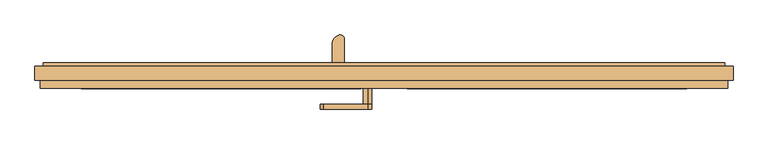
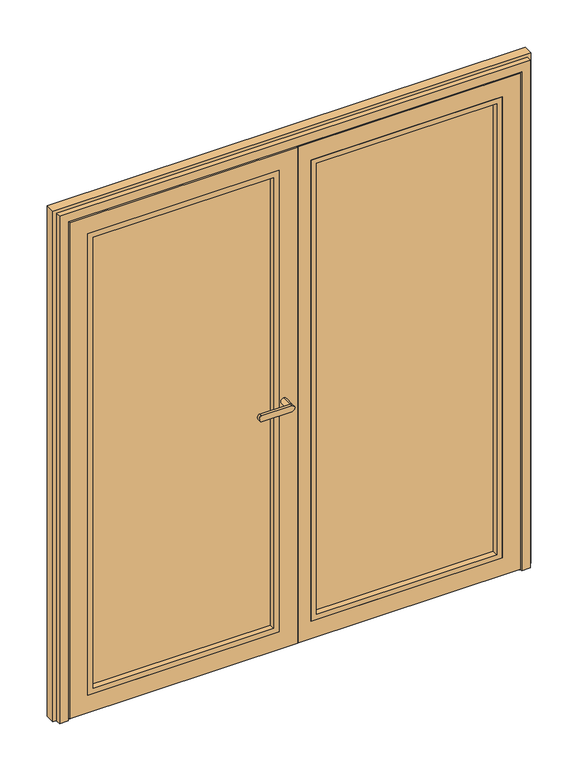
"""IFC4 building model written with IfcOpenShell, lengths in millimetres: door geometry, Schueco_FWS_ADS-70-HD_inw_Family-02 : FWS SI insert unit."""

from ifc_helpers import new_model, si_unit, point, frame, frame_2d, origin, place, context, project, spatial, polyline, circle_curve, ellipse_curve, trimmed, segment, composite_curve, outline, extrude, faceted_brep, source, transform, mapped, element, save
from ifc_brep_helpers import plane_surface, cylinder_surface, extruded_surface, advanced_brep


def door_4fc60986(model_context):
    return source(origin(), model_context, "Body", "SolidModel", [
        faceted_brep([(900.0, -52.5000065, 8.0), (900.0, -52.5000065, 2100.0), (900.0, -61.0002823, 2100.0), (900.0, -61.0002823, 8.0), (15.0, -61.0002823, 8.0), (15.0, -52.5000065, 8.0), (15.0, -52.5000065, 23.0), (885.0, -52.5000065, 23.0), (885.0, -52.5000065, 2085.0), (15.0, -52.5000065, 2085.0), (15.0, -52.5000065, 2100.0), (15.0, -61.0002823, 2100.0), (63.0, -61.0002823, 81.0), (63.0, -61.0002823, 2027.0), (827.0, -61.0002823, 2027.0), (827.0, -61.0002823, 81.0), (827.0, 0.4997603, 2027.0), (827.0, 0.4997603, 81.0), (63.0, 0.4997603, 81.0), (63.0, 0.4997603, 2027.0), (88.0, 0.4997603, 106.0), (88.0, 0.4997603, 2002.0), (802.0, 0.4997603, 2002.0), (802.0, 0.4997603, 106.0), (802.0, 8.9997177, 2002.0), (802.0, 8.9997177, 106.0), (88.0, 8.9997177, 106.0), (88.0, 8.9997177, 2002.0), (875.0, 8.9997177, 33.0), (-10.0, 8.9997177, 33.0), (-10.0, 8.9997177, 2075.0), (875.0, 8.9997177, 2075.0), (875.0, 0.4997603, 2075.0), (875.0, 0.4997603, 33.0), (5.0, 0.4997603, 33.0), (-10.0, 0.4997603, 33.0), (5.0, 0.4997603, 23.0), (5.0, 0.4997603, 2075.0), (5.0, 0.4997603, 2085.0), (885.0, 0.4997603, 2085.0), (885.0, 0.4997603, 23.0), (5.0, -52.5000065, 23.0), (5.0, -52.5000065, 2085.0), (-10.0, 0.4997603, 2075.0)], [[[0, 1, 2, 3]], [[3, 4, 5, 0]], [[0, 5, 6, 7, 8, 9, 10, 1]], [[2, 11, 4, 3], [12, 13, 14, 15]], [[15, 14, 16, 17]], [[17, 18, 12, 15]], [[18, 19, 13, 12]], [[17, 16, 19, 18], [20, 21, 22, 23]], [[23, 22, 24, 25]], [[25, 26, 20, 23]], [[26, 27, 21, 20]], [[28, 29, 30, 31], [25, 24, 27, 26]], [[28, 31, 32, 33]], [[33, 34, 35, 29, 28]], [[36, 34, 33, 32, 37, 38, 39, 40]], [[40, 39, 8, 7]], [[7, 6, 41, 36, 40]], [[41, 42, 38, 37, 34, 36]], [[1, 10, 11, 2]], [[19, 16, 14, 13]], [[27, 24, 22, 21]], [[31, 30, 43, 37, 32]], [[42, 9, 8, 39, 38]], [[6, 5, 4, 11, 10, 9]], [[35, 43, 30, 29]], [[35, 34, 37, 43]], [[9, 42, 41, 6]]]),
        extrude(outline(polyline([(81.0, 63.0), (81.0, 827.0), (2027.0, 827.0), (2027.0, 63.0), (81.0, 63.0)]), holes=[polyline([(103.0, 805.0), (103.0, 85.0), (2005.0, 85.0), (2005.0, 805.0), (103.0, 805.0)])]), frame((0.0, -61.0002823, 0.0), z_axis=(0.0, 1.0, 0.0), x_axis=(0.0, 0.0, 1.0)), (0.0, 0.0, 1.0), 23.5000426),
        extrude(outline(polyline([(63.0, -37.5002397), (63.0, 0.4997603), (827.0, 0.4997603), (827.0, -37.5002397), (63.0, -37.5002397)])), frame((0.0, 0.0, 81.0), z_axis=(0.0, 0.0, 1.0), x_axis=(1.0, 0.0, 0.0)), (0.0, 0.0, 1.0), 1946.0),
        extrude(outline(composite_curve([segment(polyline([(-26.2439405, 23.0), (-26.2439405, 4.2956275)]), True, "CONTINUOUS"), segment(trimmed(circle_curve(frame_2d((-36.8963068, 15.355415)), 15.3555139), [point((-26.2439405, 4.2956275))], [point((-47.548673, 4.2956275))], False, "CARTESIAN"), True, "CONTINUOUS"), segment(polyline([(-47.548673, 4.2956275), (-47.548673, 23.0), (-26.2439405, 23.0)]), True, "CONTINUOUS")], self_intersect=False)), frame((5.0, 0.0, 0.0), z_axis=(1.0, 0.0, 0.0), x_axis=(0.0, 1.0, 0.0)), (0.0, 0.0, 1.0), 880.0),
        extrude(outline(polyline([(875.0, 0.4997603), (-10.0, 0.4997603), (-10.0, 8.9997177), (875.0, 8.9997177), (875.0, 0.4997603)])), frame((0.0, 0.0, 8.0), z_axis=(0.0, 0.0, 1.0), x_axis=(1.0, 0.0, 0.0)), (0.0, 0.0, 1.0), 25.0),
        extrude(outline(composite_curve([segment(polyline([(-141.6673236, 8.9997177), (-141.6673236, 59.1618682)]), True, "CONTINUOUS"), segment(trimmed(circle_curve(frame_2d((-114.4889059, 59.1618682)), 27.1784177), [point((-141.6673236, 59.1618682))], [point((-124.0260015, 84.6120194))], False, "CARTESIAN"), True, "CONTINUOUS"), segment(trimmed(circle_curve(frame_2d((-119.9485005, 73.7310321)), 11.6198924), [point((-124.0260015, 84.6120194))], [point((-108.3286081, 73.7310321))], False, "CARTESIAN"), True, "CONTINUOUS"), segment(polyline([(-108.3286081, 73.7310321), (-108.3286081, 8.9997177), (-141.6673236, 8.9997177)]), True, "CONTINUOUS")], self_intersect=False)), frame((0.0, 0.0, 2043.9340013), z_axis=(0.0, 0.0, 1.0), x_axis=(1.0, 0.0, 0.0)), (0.0, 0.0, 1.0), 4.0),
        extrude(outline(polyline([(-141.6673236, 12.9997177), (-108.3286081, 12.9997177), (-108.3286081, 8.9997177), (-141.6673236, 8.9997177), (-141.6673236, 12.9997177)])), frame((0.0, 0.0, 2013.9340013), z_axis=(0.0, 0.0, 1.0), x_axis=(1.0, 0.0, 0.0)), (0.0, 0.0, 1.0), 30.0),
        extrude(outline(polyline([(-141.6673236, 12.9997177), (-108.3286081, 12.9997177), (-108.3286081, 8.9997177), (-141.6673236, 8.9997177), (-141.6673236, 12.9997177)])), frame((0.0, 0.0, 56.9340013), z_axis=(0.0, 0.0, 1.0), x_axis=(1.0, 0.0, 0.0)), (0.0, 0.0, 1.0), 30.0),
        extrude(outline(composite_curve([segment(polyline([(-141.6673236, 8.9997177), (-141.6673236, 59.1618682)]), True, "CONTINUOUS"), segment(trimmed(circle_curve(frame_2d((-114.4889059, 59.1618682)), 27.1784177), [point((-141.6673236, 59.1618682))], [point((-124.0260015, 84.6120194))], False, "CARTESIAN"), True, "CONTINUOUS"), segment(trimmed(circle_curve(frame_2d((-119.9485005, 73.7310321)), 11.6198924), [point((-124.0260015, 84.6120194))], [point((-108.3286081, 73.7310321))], False, "CARTESIAN"), True, "CONTINUOUS"), segment(polyline([(-108.3286081, 73.7310321), (-108.3286081, 8.9997177), (-141.6673236, 8.9997177)]), True, "CONTINUOUS")], self_intersect=False)), frame((0.0, 0.0, 52.9340013), z_axis=(0.0, 0.0, 1.0), x_axis=(1.0, 0.0, 0.0)), (0.0, 0.0, 1.0), 4.0),
        advanced_brep(
        [(-112.282924, 57.5977179, 2043.9340013), (-137.717076, 72.2821425, 2043.9340013), (-112.282924, 57.5977179, 56.9340013), (-137.717076, 72.2821425, 56.9340013)],
        [
            (0, 1, ellipse_curve(frame((-125.0, 64.9399302, 2043.9340013), z_axis=(0.0, 0.0, 1.0000000000000002), x_axis=(0.5000002582658958, 0.866025254674503, 0.0)), 21.5840887, 14.6844171)),
            (1, 0, ellipse_curve(frame((-125.0, 64.9399302, 2043.9340013), z_axis=(0.0, 0.0, 1.0000000000000002), x_axis=(0.5000002582658958, 0.866025254674503, 0.0)), 21.5840887, 14.6844171)),
            (2, 3, ellipse_curve(frame((-125.0, 64.9399302, 56.9340013), z_axis=(0.0, 0.0, -1.0000000000000002), x_axis=(-0.866025254674503, 0.5000002582658958, 0.0)), 14.6844171, 21.5840887)),
            (3, 2, ellipse_curve(frame((-125.0, 64.9399302, 56.9340013), z_axis=(0.0, 0.0, -1.0000000000000002), x_axis=(-0.866025254674503, 0.5000002582658958, 0.0)), 14.6844171, 21.5840887)),
            (0, 2),
            (3, 1),
        ],
        [
            plane_surface(frame((-137.717076, 72.2821425, 2043.9340013), z_axis=(0.0, 0.0, 1.0000000000000002), x_axis=(0.5000002582658958, 0.866025254674503, 0.0))),
            plane_surface(frame((-137.717076, 72.2821425, 56.9340013), z_axis=(0.0, 0.0, -1.0000000000000002), x_axis=(-0.5000002582658958, -0.866025254674503, 0.0))),
            extruded_surface(trimmed(ellipse_curve(frame((-125.0, 64.9399302, 56.9340013), z_axis=(0.0, 0.0, -1.0000000000000002), x_axis=(-0.866025254674503, 0.5000002582658958, 0.0)), 14.6844171, 21.5840887), [point((-137.717076, 72.2821425, 56.9340013))], [point((-112.282924, 57.5977179, 56.9340013))], True, "CARTESIAN"), (0.0, 0.0, -1987.0), 1987.0),
            extruded_surface(trimmed(ellipse_curve(frame((-125.0, 64.9399302, 56.9340013), z_axis=(0.0, 0.0, -1.0000000000000002), x_axis=(-0.866025254674503, 0.5000002582658958, 0.0)), 14.6844171, 21.5840887), [point((-112.282924, 57.5977179, 56.9340013))], [point((-137.717076, 72.2821425, 56.9340013))], True, "CARTESIAN"), (0.0, 0.0, -1987.0), 1987.0),
        ],
        [
            (0, [[1, 2]]),
            (1, [[3, 4]]),
            (2, [[5, -4, 6, -1]]),
            (3, [[-6, -3, -5, -2]]),
        ],
    ),
        advanced_brep(
        [(-45.0, -117.0002518, 1038.0113692), (-45.0, -117.0002518, 1061.9886308), (-166.6617926, -117.0002518, 1061.9886308), (-166.6617926, -117.0002518, 1038.0113692), (-45.0, -104.5001648, 1061.9886308), (-45.0, -104.5001648, 1038.0113692), (-166.6617926, -104.5001648, 1038.0113692), (-166.6617926, -104.5001648, 1061.9886308), (-45.0, -61.0002823, 1038.0113692), (-45.0, -61.0002823, 1061.9886308)],
        [
            (0, 1, circle_curve(frame((-45.0, -117.0002518, 1050.0), z_axis=(0.0, -1.0, 0.0), x_axis=(0.0, 0.0, 1.0)), 11.9886308)),
            (1, 2),
            (2, 3, ellipse_curve(frame((-166.6617926, -117.0002518, 1050.0), z_axis=(0.0, -1.0, 0.0), x_axis=(0.0, 0.0, -1.0)), 11.9886308, 7.9050795)),
            (3, 0),
            (4, 5, circle_curve(frame((-45.0, -104.5001648, 1050.0), z_axis=(0.0, -1.0, 0.0), x_axis=(0.0, 0.0, 1.0)), 11.9886308)),
            (5, 6),
            (6, 7, ellipse_curve(frame((-166.6617926, -104.5001648, 1050.0), z_axis=(0.0, 1.0, 0.0), x_axis=(0.0, 0.0, -1.0)), 11.9886308, 7.9050795)),
            (7, 4),
            (3, 6),
            (5, 0),
            (2, 7),
            (1, 4),
            (5, 4, circle_curve(frame((-45.0, -104.5001648, 1050.0), z_axis=(0.0, -1.0, 0.0), x_axis=(0.0, 0.0, 1.0)), 11.9886308)),
            (8, 9, circle_curve(frame((-45.0, -61.0002823, 1050.0), z_axis=(0.0, 1.0, 0.0), x_axis=(0.0, 0.0, 1.0)), 11.9886308)),
            (9, 8, circle_curve(frame((-45.0, -61.0002823, 1050.0), z_axis=(0.0, 1.0, 0.0), x_axis=(0.0, 0.0, 1.0)), 11.9886308)),
            (8, 5),
            (4, 9),
        ],
        [
            plane_surface(frame((-166.6617926, -117.0002518, 1038.0113692), z_axis=(0.0, -1.0, 0.0), x_axis=(-1.0, 0.0, 0.0))),
            plane_surface(frame((-166.6617926, -104.5001648, 1038.0113692), z_axis=(0.0, 1.0, 0.0), x_axis=(1.0, 0.0, 0.0))),
            plane_surface(frame((-45.0, -117.0002518, 1038.0113692), z_axis=(0.0, 0.0, -1.0), x_axis=(0.0, 1.0, 0.0))),
            extruded_surface(trimmed(ellipse_curve(frame((-166.6617926, -104.5001648, 1050.0), z_axis=(0.0, 1.0, 0.0), x_axis=(0.0, 0.0, -1.0)), 11.9886308, 7.9050795), [point((-166.6617926, -104.5001648, 1038.0113692))], [point((-166.6617926, -104.5001648, 1061.9886308))], True, "CARTESIAN"), (0.0, 12.500086999999994, 0.0), 12.500086999999994),
            plane_surface(frame((-166.6617926, -117.0002518, 1061.9886308), z_axis=(0.0, 0.0, 1.0), x_axis=(0.0, 1.0, 0.0))),
            cylinder_surface(frame((-45.0, -104.5001648, 1050.0), z_axis=(0.0, -1.0, 0.0), x_axis=(0.0, 0.0, 1.0)), 11.9886308),
            plane_surface(frame((-45.0, -61.0002823, 1061.9886308), z_axis=(0.0, 1.0, 0.0), x_axis=(-1.0, 0.0, 0.0))),
            cylinder_surface(frame((-45.0, -61.0002823, 1050.0), z_axis=(0.0, -1.0, 0.0), x_axis=(0.0, 0.0, 1.0)), 11.9886308),
        ],
        [
            (0, [[1, 2, 3, 4]]),
            (1, [[5, 6, 7, 8]]),
            (2, [[9, -6, 10, -4]]),
            (3, [[11, -7, -9, -3]]),
            (4, [[12, -8, -11, -2]]),
            (5, [[-10, 13, -12, -1]]),
            (6, [[14, 15]]),
            (7, [[16, -5, 17, -14]]),
            (7, [[-17, -13, -16, -15]]),
        ],
    ),
        faceted_brep([(-900.0, -52.5000065, 8.0), (-900.0, -61.0002823, 8.0), (-900.0, -61.0002823, 2100.0), (-900.0, -52.5000065, 2100.0), (10.0, -52.5000065, 8.0), (10.0, -61.0002823, 8.0), (10.0, -52.5000065, 2100.0), (-885.0, -52.5000065, 23.0), (-5.0, -52.5000065, 23.0), (-5.0, -52.5000065, 2085.0), (-885.0, -52.5000065, 2085.0), (10.0, -61.0002823, 2100.0), (-63.0, -61.0002823, 81.0), (-827.0, -61.0002823, 81.0), (-827.0, -61.0002823, 2027.0), (-63.0, -61.0002823, 2027.0), (-827.0, 0.4997603, 81.0), (-827.0, 0.4997603, 2027.0), (-63.0, 0.4997603, 81.0), (-63.0, 0.4997603, 2027.0), (-88.0, 0.4997603, 106.0), (-802.0, 0.4997603, 106.0), (-802.0, 0.4997603, 2002.0), (-88.0, 0.4997603, 2002.0), (-802.0, 8.9997177, 106.0), (-802.0, 8.9997177, 2002.0), (-88.0, 8.9997177, 106.0), (-88.0, 8.9997177, 2002.0), (-15.0, 8.9997177, 2075.0), (-15.0, 8.9997177, 33.0), (-25.0, 8.9997177, 33.0), (-875.0, 8.9997177, 33.0), (-875.0, 8.9997177, 2075.0), (-25.0, 8.9997177, 2075.0), (-875.0, 0.4997603, 33.0), (-875.0, 0.4997603, 2075.0), (-15.0, 0.4997603, 33.0), (-25.0, 0.4997603, 33.0), (-15.0, 0.4997603, 2075.0), (-5.0, 0.4997603, 23.0), (-885.0, 0.4997603, 23.0), (-885.0, 0.4997603, 2085.0), (-5.0, 0.4997603, 2085.0), (-25.0, 0.4997603, 2075.0)], [[[0, 1, 2, 3]], [[1, 0, 4, 5]], [[4, 0, 3, 6], [7, 8, 9, 10]], [[5, 4, 6, 11]], [[1, 5, 11, 2], [12, 13, 14, 15]], [[13, 16, 17, 14]], [[16, 13, 12, 18]], [[18, 12, 15, 19]], [[16, 18, 19, 17], [20, 21, 22, 23]], [[21, 24, 25, 22]], [[24, 21, 20, 26]], [[26, 20, 23, 27]], [[28, 29, 30, 31, 32, 33], [24, 26, 27, 25]], [[31, 34, 35, 32]], [[34, 31, 30, 29, 36, 37]], [[36, 29, 28, 38]], [[39, 40, 41, 42], [36, 38, 43, 35, 34, 37]], [[40, 7, 10, 41]], [[7, 40, 39, 8]], [[8, 39, 42, 9]], [[11, 6, 3, 2]], [[19, 15, 14, 17]], [[27, 23, 22, 25]], [[38, 28, 33, 32, 35, 43]], [[9, 42, 41, 10]]]),
        extrude(outline(polyline([(81.0, -63.0), (2027.0, -63.0), (2027.0, -827.0), (81.0, -827.0), (81.0, -63.0)]), holes=[polyline([(103.0, -805.0), (2005.0, -805.0), (2005.0, -85.0), (103.0, -85.0), (103.0, -805.0)])]), frame((0.0, -61.0002823, 0.0), z_axis=(0.0, 1.0, 0.0), x_axis=(0.0, 0.0, 1.0)), (0.0, 0.0, 1.0), 23.5000426),
        extrude(outline(polyline([(-63.0, -37.5002397), (-827.0, -37.5002397), (-827.0, 0.4997603), (-63.0, 0.4997603), (-63.0, -37.5002397)])), frame((0.0, 0.0, 81.0), z_axis=(0.0, 0.0, 1.0), x_axis=(1.0, 0.0, 0.0)), (0.0, 0.0, 1.0), 1946.0),
        extrude(outline(composite_curve([segment(polyline([(-26.2439405, 23.0), (-26.2439405, 4.2956275)]), True, "CONTINUOUS"), segment(trimmed(circle_curve(frame_2d((-36.8963068, 15.355415)), 15.3555139), [point((-26.2439405, 4.2956275))], [point((-47.548673, 4.2956275))], False, "CARTESIAN"), True, "CONTINUOUS"), segment(polyline([(-47.548673, 4.2956275), (-47.548673, 23.0), (-26.2439405, 23.0)]), True, "CONTINUOUS")], self_intersect=False)), frame((-885.0, 0.0, 0.0), z_axis=(1.0, 0.0, 0.0), x_axis=(0.0, 1.0, 0.0)), (0.0, 0.0, 1.0), 880.0),
        extrude(outline(polyline([(-875.0, 0.4997603), (-875.0, 8.9997177), (-15.0, 8.9997177), (-15.0, 0.4997603), (-875.0, 0.4997603)])), frame((0.0, 0.0, 8.0), z_axis=(0.0, 0.0, 1.0), x_axis=(1.0, 0.0, 0.0)), (0.0, 0.0, 1.0), 25.0),
        faceted_brep([(930.999943, 8.9997177, 2130.999943), (930.999943, 0.0, 2130.999943), (930.999943, 0.0, 0.0), (930.999943, 8.9997177, 0.0), (-954.0, 0.0, 0.0), (-954.0, 0.0, 2154.0), (954.0, 0.0, 2154.0), (954.0, 0.0, 0.0), (-930.999943, 0.0, 2130.999943), (-930.999943, 0.0, 0.0), (954.0, -38.0, 0.0), (940.0, -38.0, 0.0), (940.0, -61.0002823, 0.0), (904.9999114, -61.0002823, 0.0), (904.9999114, -52.5000065, 0.0), (893.4999114, -52.5000065, 0.0), (893.4999114, 0.4997603, 0.0), (879.9999888, 0.4997603, 0.0), (879.9999888, 8.9997177, 0.0), (-879.9999888, 8.9997177, 0.0), (-930.999943, 8.9997177, 0.0), (-930.999943, 8.9997177, 2130.999943), (879.9999888, 8.9997177, 2079.9999888), (-879.9999888, 8.9997177, 2079.9999888), (904.9999114, -61.0002823, 2104.9999114), (904.9999114, -52.5000065, 2104.9999114), (-904.9999114, -52.5000065, 0.0), (-893.4999114, -52.5000065, 0.0), (-893.4999114, -52.5000065, 2093.4999114), (893.4999114, -52.5000065, 2093.4999114), (-904.9999114, -52.5000065, 2104.9999114), (-940.0, -61.0002823, 0.0), (-904.9999114, -61.0002823, 0.0), (-904.9999114, -61.0002823, 2104.9999114), (940.0, -61.0002823, 2140.0), (-940.0, -61.0002823, 2140.0), (940.0, -38.0, 2140.0), (-954.0, -38.0, 0.0), (-940.0, -38.0, 0.0), (-940.0, -38.0, 2140.0), (954.0, -38.0, 2154.0), (-954.0, -38.0, 2154.0), (-879.9999888, 0.4997603, 0.0), (-893.4999114, 0.4997603, 0.0), (879.9999888, 0.4997603, 2079.9999888), (-879.9999888, 0.4997603, 2079.9999888), (893.4999114, 0.4997603, 2093.4999114), (-893.4999114, 0.4997603, 2093.4999114)], [[[0, 1, 2, 3]], [[4, 5, 6, 7, 2, 1, 8, 9]], [[3, 2, 7, 10, 11, 12, 13, 14, 15, 16, 17, 18]], [[19, 20, 21, 0, 3, 18, 22, 23]], [[24, 25, 14, 13]], [[26, 27, 28, 29, 15, 14, 25, 30]], [[31, 32, 33, 24, 13, 12, 34, 35]], [[34, 12, 11, 36]], [[37, 38, 39, 36, 11, 10, 40, 41]], [[4, 9, 20, 19, 42, 43, 27, 26, 32, 31, 38, 37]], [[20, 9, 8, 21]], [[18, 17, 44, 22]], [[42, 19, 23, 45]], [[32, 26, 30, 33]], [[31, 35, 39, 38]], [[4, 37, 41, 5]], [[6, 40, 10, 7]], [[43, 42, 45, 44, 17, 16, 46, 47]], [[16, 15, 29, 46]], [[27, 43, 47, 28]], [[21, 8, 1, 0]], [[33, 30, 25, 24]], [[35, 34, 36, 39]], [[23, 22, 44, 45]], [[5, 41, 40, 6]], [[47, 46, 29, 28]]]),
    ])


if __name__ == "__main__":
    model = new_model("IFC4")
    model_context = context("Model", 3, world=origin())
    ifc_project = project(units=[si_unit("LENGTHUNIT", "METRE", prefix="MILLI")], contexts=[model_context])
    site = spatial("IfcSite", under=ifc_project)
    building = spatial("IfcBuilding", under=site)
    placement = place(None, origin())
    door_shape = door_4fc60986(model_context)
    element("IfcDoor", 1, ObjectType="Schueco_FWS_ADS-70-HD_inw_Family-02 : FWS SI insert unit", at=placement, inside=building, context=model_context, shape_type="MappedRepresentation", body=[
        mapped(door_shape, transform((0.0, 0.0, 0.0), x_axis=(1.0, 0.0, 0.0), y_axis=(0.0, 1.0, 0.0), z_axis=(0.0, 0.0, 1.0))),
    ])
    save(model, "model.ifc")

# Revit data of these elements
# Type "Schueco_FWS_ADS-70-HD_inw_Family-02 : FWS SI insert unit"
#   Type Mark = "42"
#   __NOTE__ = "Data describes the optimum values of the entire system. The properites of a selected design option have to be determined on an individual basis!"
#   Wind load resistance = "Class 2"
#   Watertightness = "Class 5A"
#   Thermal insulation = "Uf = 1.6 W/(m²K)"
#   Sound insulation = "to Rw 43 dB"
#   Schueco thermal insulation standard = "Thermally insulated"
#   Opening type = "Inward-opening, Flush-fitted"
#   Model = "Schueco ADS 70 HD"
#   Mechanical loading = "Class 2"
#   Maximum leaf width in mm = "1400"
#   Maximum leaf weight in kg = "200"
#   Maximum leaf height in mm = "3000"
#   Material = "Aluminium"
#   Long term functionality = "Class 6"
#   Construction Type = "Door, double-leaf, inward-opening"
#   Manufacturer = "Schueco International KG"
#   Glazing data = "Triple glazing 38mm"
#   Façade insert unit = "yes"
#   Family creation date = "08.2017"
#   Description = "Schueco Aluminium Door System (ADS)"
#   Burglar resistance = "Class RC 3"
#   Areas of use = "Public buildings"
#   Analytic Construction = "<None>"
#   Air permeability = "Class 2"
#   Width [instance default] = 1658.817 mm
#   Leaf opening angle [instance default] = 0.00°
#   IOf_T = 38 mm
#   Height [instance default] = 2117.739 mm
#   Glazing area [instance default] = 2.19229 m²
#   F2_W [instance default] = 829.409 mm
#   F1_W [instance default] = 829.409 mm
#   Distance from bottom to handles [instance default] = 1050 mm
#   Clear opening width [instance default] = 1510.817 mm
#   Active leaf width = 1100 mm
#   Standard threshold = no
#   Low level threshold = yes
#   Handles = yes
#   FWS SI insert unit = yes
#   FWS HI insert unit = no
#   All fields of identical width = yes
#   Glass = none
#   Frame = Alu
#   Fittings = none
# Element 1 (IfcDoor, "Schueco_FWS_ADS-70-HD_inw_Family-02 : FWS SI insert unit")
#   Width = 1908 mm
#   Height = 2154 mm
#   Glazing area = 2.70749 m²
#   F2_W = 954 mm
#   F1_W = 954 mm
#   Clear opening width = 1760 mm
#   Materials on its faces: "Alu", "Glass"
# Materials
#   "Alu": class "Glas", colour RGB 140 140 140, transparency 0
#   "Glass": class "Glass", colour RGB 128 128 255, transparency 0.75, Description = "Soda Lime Glass", Cost = 0
